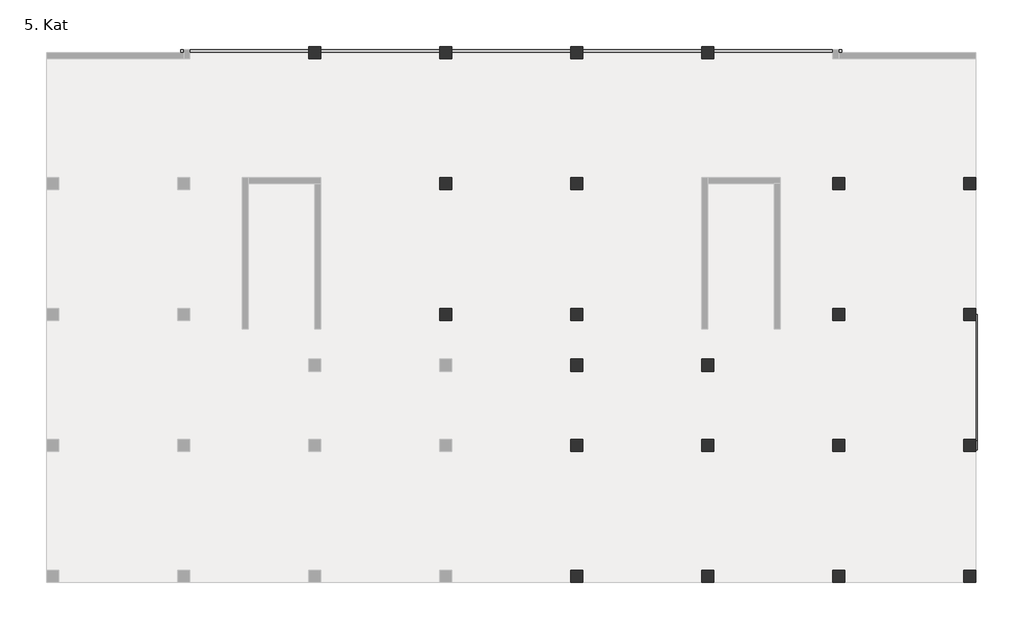
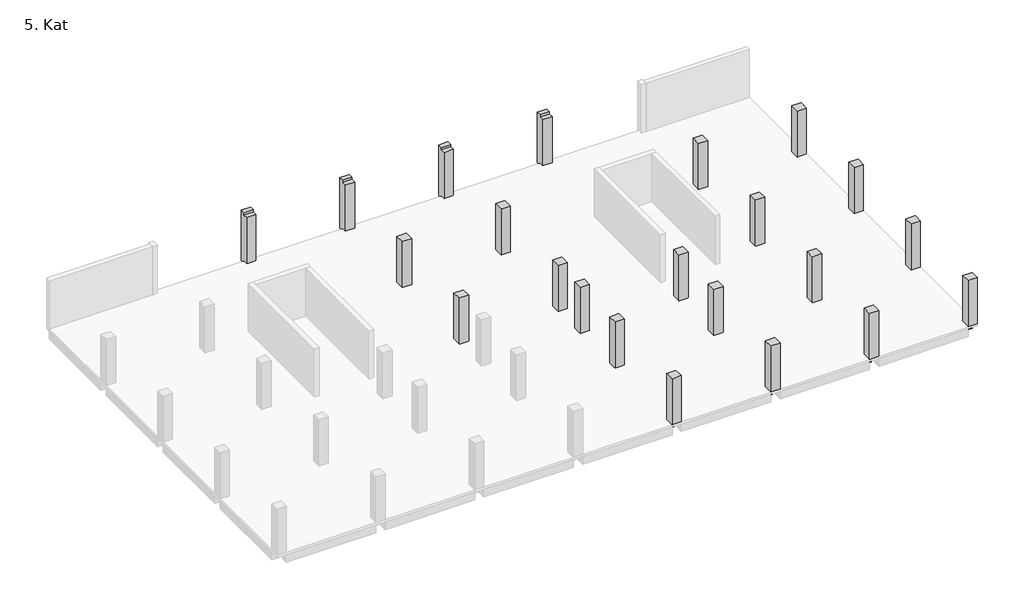
# One storey, part 2 of 2: 46 beams, 22 columns.
"""IFC4 building model written with IfcOpenShell, lengths in millimetres."""

from ifc_helpers import new_model, si_unit, frame, origin, place, context, project, spatial, polyline, outline, extrude, faceted_brep, element, save

model = new_model("IFC4")

# Units and contexts
model_context = context("Model", 3, world=origin())
ifc_project = project(units=[si_unit("LENGTHUNIT", "METRE", prefix="MILLI")], contexts=[model_context])

# Site, building, storey
site = spatial("IfcSite", under=ifc_project)
building = spatial("IfcBuilding", under=site)
storey = spatial("IfcBuildingStorey", under=building, Name="5. Kat", Elevation=26500.0)

# Beams
placement = place(None, origin())
element("IfcBeam", 1, ObjectType="M_Concrete-Rectangular Beam : 60x70cm kiriş", at=placement, inside=storey, context=model_context, shape_type="Brep", body=[
    faceted_brep([(8899.9995273, 34200.0000099, 26500.0), (8899.9993907, 33600.0000099, 26500.0), (16599.9993907, 33600.0000099, 26500.0), (16599.9993907, 34200.0000099, 26500.0), (8899.9993907, 33600.0000099, 25800.0), (16599.9993907, 33600.0000099, 25800.0), (8899.9995273, 34200.0000099, 25800.0), (16599.9993907, 34200.0000099, 25800.0)], [[[0, 1, 2, 3]], [[1, 4, 5, 2]], [[4, 6, 7, 5]], [[3, 7, 6, 0]], [[0, 6, 4, 1]], [[3, 2, 5, 7]]]),
])
element("IfcBeam", 2, ObjectType="M_Concrete-Rectangular Beam : 60x70cm kiriş", at=placement, inside=storey, context=model_context, shape_type="SweptSolid", body=[
    extrude(outline(polyline([(25099.9993907, 34200.0000277), (25099.9993907, 33600.0000277), (17399.9993907, 33600.0000277), (17399.9993907, 34200.0000277), (25099.9993907, 34200.0000277)])), frame((0.0, 0.0, 25800.0), z_axis=(0.0, 0.0, 1.0), x_axis=(1.0, 0.0, 0.0)), (0.0, 0.0, 1.0), 700.0),
])
element("IfcBeam", 3, ObjectType="M_Concrete-Rectangular Beam : 60x70cm kiriş", at=placement, inside=storey, context=model_context, shape_type="SweptSolid", body=[
    extrude(outline(polyline([(33599.9993907, 34200.000044), (33599.9993907, 33600.000044), (25899.9993907, 33600.000044), (25899.9993907, 34200.000044), (33599.9993907, 34200.000044)])), frame((0.0, 0.0, 25800.0), z_axis=(0.0, 0.0, 1.0), x_axis=(1.0, 0.0, 0.0)), (0.0, 0.0, 1.0), 700.0),
])
element("IfcBeam", 4, ObjectType="M_Concrete-Rectangular Beam : 60x70cm kiriş", at=placement, inside=storey, context=model_context, shape_type="SweptSolid", body=[
    extrude(outline(polyline([(34399.9993907, 33600.0000618), (34399.9993907, 34200.0000618), (42099.9993899, 34200.0000618), (42099.9993899, 33600.0000618), (34399.9993907, 33600.0000618)])), frame((0.0, 0.0, 25800.0), z_axis=(0.0, 0.0, 1.0), x_axis=(1.0, 0.0, 0.0)), (0.0, 0.0, 1.0), 700.0),
])
element("IfcBeam", 5, ObjectType="M_Concrete-Rectangular Beam : 60x70cm kiriş", at=placement, inside=storey, context=model_context, shape_type="Brep", body=[
    faceted_brep([(42899.999681, 34200.0000788, 26500.0), (42899.999681, 33600.0000788, 26500.0), (50599.9994944, 33600.0000788, 26500.0), (50599.9994944, 34000.0004303, 26500.0), (50599.9994944, 34193.7257565, 26500.0), (50999.9994944, 34193.7257565, 26500.0), (50999.9994944, 34200.0000788, 26500.0), (42899.999681, 34200.0000788, 25800.0), (50999.9994944, 34200.0000788, 25800.0), (42899.999681, 33600.0000788, 25800.0), (50999.9994944, 34193.7257565, 25800.0), (50599.9994944, 34193.7257565, 25800.0), (50599.9994944, 34000.0004303, 25800.0), (50599.9994944, 33600.0000788, 25800.0)], [[[0, 1, 2, 3, 4, 5, 6]], [[7, 0, 6, 8]], [[9, 7, 8, 10, 11, 12, 13]], [[1, 9, 13, 2]], [[1, 0, 7, 9]], [[8, 6, 5, 10]], [[11, 4, 3, 2, 13, 12]], [[4, 11, 10, 5]]]),
])
element("IfcBeam", 6, ObjectType="M_Concrete-Rectangular Beam : 60x70cm kiriş", at=placement, inside=storey, context=model_context, shape_type="Brep", body=[
    faceted_brep([(17399.9996817, 33600.0009197, 26500.0), (16799.9996817, 33600.0009197, 26500.0), (16799.9996817, 25900.0003816, 26500.0), (16999.9995362, 25900.0003816, 26500.0), (17399.9996817, 25900.0003816, 26500.0), (17399.9996817, 33600.0009197, 25800.0), (17399.9996817, 25900.0003816, 25800.0), (16799.9996817, 33600.0009197, 25800.0), (16799.9996817, 25900.0003816, 25800.0)], [[[0, 1, 2, 3, 4]], [[5, 0, 4, 6]], [[7, 5, 6, 8]], [[1, 7, 8, 2]], [[0, 5, 7, 1]], [[4, 3, 2, 8, 6]]]),
])
element("IfcBeam", 7, ObjectType="M_Concrete-Rectangular Beam : 60x70cm kiriş", at=placement, inside=storey, context=model_context, shape_type="SweptSolid", body=[
    extrude(outline(polyline([(25899.9996503, 25900.0004105), (25299.9996503, 25900.0004105), (25299.9996503, 33600.0009197), (25899.9996503, 33600.0009197), (25899.9996503, 25900.0004105)])), frame((0.0, 0.0, 25800.0), z_axis=(0.0, 0.0, 1.0), x_axis=(1.0, 0.0, 0.0)), (0.0, 0.0, 1.0), 700.0),
])
element("IfcBeam", 8, ObjectType="M_Concrete-Rectangular Beam : 60x70cm kiriş", at=placement, inside=storey, context=model_context, shape_type="Brep", body=[
    faceted_brep([(17399.9996817, 25900.0000279, 26500.0), (17399.9995847, 25500.0003816, 26500.0), (17399.9995362, 25300.0000279, 26500.0), (25099.9993907, 25300.0000279, 26500.0), (25099.9993907, 25900.0000279, 26500.0), (17399.9996817, 25900.0000279, 25800.0), (25099.9993907, 25900.0000279, 25800.0), (17399.9995362, 25300.0000279, 25800.0), (25099.9993907, 25300.0000279, 25800.0)], [[[0, 1, 2, 3, 4]], [[5, 0, 4, 6]], [[7, 5, 6, 8]], [[8, 3, 2, 7]], [[0, 5, 7, 2, 1]], [[3, 8, 6, 4]]]),
])
element("IfcBeam", 9, ObjectType="M_Concrete-Rectangular Beam : 40x70cm kiriş 2", at=placement, inside=storey, context=model_context, shape_type="SweptSolid", body=[
    extrude(outline(polyline([(25099.999715, 17400.0003766), (25099.999715, 17000.0003766), (17399.9995362, 17000.0003766), (17399.9995362, 17400.0003766), (25099.999715, 17400.0003766)])), frame((0.0, 0.0, 25800.0), z_axis=(0.0, 0.0, 1.0), x_axis=(1.0, 0.0, 0.0)), (0.0, 0.0, 1.0), 700.0),
])
element("IfcBeam", 10, ObjectType="M_Concrete-Rectangular Beam : 60x70cm kiriş", at=placement, inside=storey, context=model_context, shape_type="SweptSolid", body=[
    extrude(outline(polyline([(25299.999682, 25099.9999518), (25899.999682, 25099.9999518), (25899.999682, 17400.0009197), (25299.999682, 17400.0009197), (25299.999682, 25099.9999518)])), frame((0.0, 0.0, 25800.0), z_axis=(0.0, 0.0, 1.0), x_axis=(1.0, 0.0, 0.0)), (0.0, 0.0, 1.0), 700.0),
])
element("IfcBeam", 11, ObjectType="M_Concrete-Rectangular Beam : 60x70cm kiriş", at=placement, inside=storey, context=model_context, shape_type="Brep", body=[
    faceted_brep([(25899.9996503, 25900.0003995, 26500.0), (25899.9993907, 25300.0003995, 26500.0), (33599.9993907, 25300.0003995, 26500.0), (33599.9993907, 25900.0003995, 26500.0), (25899.9996503, 25900.0003995, 25800.0), (33599.9993907, 25900.0003995, 25800.0), (25899.9993907, 25300.0003995, 25800.0), (33599.9993907, 25300.0003995, 25800.0)], [[[0, 1, 2, 3]], [[4, 0, 3, 5]], [[6, 4, 5, 7]], [[1, 6, 7, 2]], [[0, 4, 6, 1]], [[3, 2, 7, 5]]]),
])
element("IfcBeam", 12, ObjectType="M_Concrete-Rectangular Beam : 60x70cm kiriş", at=placement, inside=storey, context=model_context, shape_type="Brep", body=[
    faceted_brep([(34199.9994248, 33600.0009197, 26500.0), (33599.9994248, 33600.000044, 26500.0), (33599.9994248, 25900.0003995, 26500.0), (34199.9994248, 25900.0004105, 26500.0), (33599.9994248, 33600.000044, 25800.0), (33599.9994248, 25900.0003995, 25800.0), (34199.9994248, 33600.0009197, 25800.0), (34199.9994248, 25900.0004105, 25800.0)], [[[0, 1, 2, 3]], [[1, 4, 5, 2]], [[4, 6, 7, 5]], [[3, 7, 6, 0]], [[0, 6, 4, 1]], [[2, 5, 7, 3]]]),
])
element("IfcBeam", 13, ObjectType="M_Concrete-Rectangular Beam : 60x70cm kiriş", at=placement, inside=storey, context=model_context, shape_type="Brep", body=[
    faceted_brep([(34399.9993907, 25900.0004179, 26500.0), (34399.9993907, 25300.0004179, 26500.0), (42099.9995162, 25300.0004179, 26500.0), (42099.9995162, 25500.0004459, 26500.0), (42099.9995162, 25900.0004179, 26500.0), (34399.9993907, 25300.0004179, 25800.0), (42099.9995162, 25300.0004179, 25800.0), (34399.9993907, 25900.0004179, 25800.0), (42099.9995162, 25900.0004179, 25800.0)], [[[0, 1, 2, 3, 4]], [[1, 5, 6, 2]], [[5, 7, 8, 6]], [[7, 0, 4, 8]], [[5, 1, 0, 7]], [[4, 3, 2, 6, 8]]]),
])
element("IfcBeam", 14, ObjectType="M_Concrete-Rectangular Beam : 60x70cm kiriş", at=placement, inside=storey, context=model_context, shape_type="Brep", body=[
    faceted_brep([(42099.9994393, 25900.0004179, 26500.0), (42499.9995162, 25900.0004366, 26500.0), (42699.9994393, 25900.0004459, 26500.0), (42699.9994393, 33600.0009197, 26500.0), (42099.9994393, 33600.0000618, 26500.0), (42099.9994393, 25900.0004179, 25800.0), (42099.9994393, 33600.0000618, 25800.0), (42699.9994393, 25900.0004459, 25800.0), (42699.9994393, 33600.0009197, 25800.0)], [[[0, 1, 2, 3, 4]], [[5, 0, 4, 6]], [[7, 5, 6, 8]], [[8, 3, 2, 7]], [[0, 5, 7, 2, 1]], [[6, 4, 3, 8]]]),
])
element("IfcBeam", 15, ObjectType="M_Concrete-Rectangular Beam : 60x70cm kiriş", at=placement, inside=storey, context=model_context, shape_type="Brep", body=[
    faceted_brep([(50599.9993899, 25300.0004722, 26500.0), (50599.9993899, 25900.0004722, 26500.0), (47199.999381, 25900.0004722, 26500.0), (47199.999381, 25500.0004459, 26500.0), (47199.999381, 25300.0004722, 26500.0), (50599.9993899, 25900.0004722, 25800.0), (47199.999381, 25900.0004722, 25800.0), (50599.9993899, 25300.0004722, 25800.0), (47199.999381, 25300.0004722, 25800.0)], [[[0, 1, 2, 3, 4]], [[1, 5, 6, 2]], [[5, 7, 8, 6]], [[7, 0, 4, 8]], [[5, 1, 0, 7]], [[8, 4, 3, 2, 6]]]),
])
element("IfcBeam", 16, ObjectType="M_Concrete-Rectangular Beam : 60x70cm kiriş", at=placement, inside=storey, context=model_context, shape_type="Brep", body=[
    faceted_brep([(51199.9994348, 33600.0004303, 26500.0), (50999.9994944, 33600.0003131, 26500.0), (50599.9994348, 33600.0000788, 26500.0), (50599.9994348, 25900.0004722, 26500.0), (51199.9994348, 25899.9999188, 26500.0), (51199.9994348, 25899.9999188, 25800.0), (51199.9994348, 33600.0004303, 25800.0), (50599.9994348, 33600.0000788, 25800.0), (50599.9994348, 25900.0004722, 25800.0)], [[[0, 1, 2, 3, 4]], [[4, 5, 6, 0]], [[7, 6, 5, 8]], [[2, 7, 8, 3]], [[0, 6, 7, 2, 1]], [[3, 8, 5, 4]]]),
])
element("IfcBeam", 17, ObjectType="M_Concrete-Rectangular Beam : 60x70cm kiriş", at=placement, inside=storey, context=model_context, shape_type="SweptSolid", body=[
    extrude(outline(polyline([(59100.0000836, 25900.0000972), (59100.0000836, 25300.0000972), (51399.9996879, 25300.0000972), (51399.9996879, 25900.0000972), (59100.0000836, 25900.0000972)])), frame((0.0, 0.0, 25800.0), z_axis=(0.0, 0.0, 1.0), x_axis=(1.0, 0.0, 0.0)), (0.0, 0.0, 1.0), 700.0),
])
element("IfcBeam", 18, ObjectType="M_Concrete-Rectangular Beam : 60x70cm kiriş", at=placement, inside=storey, context=model_context, shape_type="SweptSolid", body=[
    extrude(outline(polyline([(59899.9996867, 25900.0004522), (59299.9996867, 25900.0004522), (59299.9996867, 33600.0004303), (59899.9996867, 33600.0004303), (59899.9996867, 25900.0004522)])), frame((0.0, 0.0, 25800.0), z_axis=(0.0, 0.0, 1.0), x_axis=(1.0, 0.0, 0.0)), (0.0, 0.0, 1.0), 700.0),
])
element("IfcBeam", 19, ObjectType="M_Concrete-Rectangular Beam : 60x70cm kiriş", at=placement, inside=storey, context=model_context, shape_type="SweptSolid", body=[
    extrude(outline(polyline([(33599.9994953, 25100.0004105), (34199.9994953, 25100.0004105), (34199.9994953, 17400.0009197), (33599.9994953, 17400.0009197), (33599.9994953, 25100.0004105)])), frame((0.0, 0.0, 25800.0), z_axis=(0.0, 0.0, 1.0), x_axis=(1.0, 0.0, 0.0)), (0.0, 0.0, 1.0), 700.0),
])
element("IfcBeam", 20, ObjectType="M_Concrete-Rectangular Beam : 40x70cm kiriş 2", at=placement, inside=storey, context=model_context, shape_type="Brep", body=[
    faceted_brep([(25899.999682, 17400.0007711, 26500.0), (25899.9993907, 17000.0007711, 26500.0), (33599.9993907, 17000.0007711, 26500.0), (33599.9994953, 17400.0007711, 26500.0), (33599.9993907, 17000.0007711, 25800.0), (25899.9993907, 17000.0007711, 25800.0), (25899.999682, 17400.0007711, 25800.0), (33599.9994953, 17400.0007711, 25800.0)], [[[0, 1, 2, 3]], [[4, 2, 1, 5]], [[5, 6, 7, 4]], [[6, 0, 3, 7]], [[0, 6, 5, 1]], [[7, 3, 2, 4]]]),
])
element("IfcBeam", 21, ObjectType="M_Concrete-Rectangular Beam : 40x70cm kiriş 2", at=placement, inside=storey, context=model_context, shape_type="SweptSolid", body=[
    extrude(outline(polyline([(42499.9995162, 14100.0003816), (42099.9995162, 14100.0003816), (42099.9995162, 16050.0004138), (42499.9995162, 16050.0004138), (42499.9995162, 14100.0003816)])), frame((0.0, 0.0, 25800.0), z_axis=(0.0, 0.0, 1.0), x_axis=(1.0, 0.0, 0.0)), (0.0, 0.0, 1.0), 700.0),
])
element("IfcBeam", 22, ObjectType="M_Concrete-Rectangular Beam : 40x70cm kiriş 2", at=placement, inside=storey, context=model_context, shape_type="SweptSolid", body=[
    extrude(outline(polyline([(34399.9997415, 13300.0003995), (34399.9997415, 13700.0003995), (41999.9997966, 13700.0003995), (41999.9997966, 13300.0003995), (34399.9997415, 13300.0003995)])), frame((0.0, 0.0, 25800.0), z_axis=(0.0, 0.0, 1.0), x_axis=(1.0, 0.0, 0.0)), (0.0, 0.0, 1.0), 700.0),
])
element("IfcBeam", 23, ObjectType="M_Concrete-Rectangular Beam : 40x70cm kiriş 2", at=placement, inside=storey, context=model_context, shape_type="SweptSolid", body=[
    extrude(outline(polyline([(34399.9993907, 17000.0007895), (34399.9993907, 17400.0007895), (42099.9995162, 17400.0007895), (42099.9995162, 17000.0007895), (34399.9993907, 17000.0007895)])), frame((0.0, 0.0, 25800.0), z_axis=(0.0, 0.0, 1.0), x_axis=(1.0, 0.0, 0.0)), (0.0, 0.0, 1.0), 700.0),
])
element("IfcBeam", 24, ObjectType="M_Concrete-Rectangular Beam : 40x70cm kiriş 2", at=placement, inside=storey, context=model_context, shape_type="SweptSolid", body=[
    extrude(outline(polyline([(42499.9995162, 17000.0003766), (42499.9995162, 17400.0003766), (46799.999381, 17400.0003766), (46799.999381, 17000.0003766), (42499.9995162, 17000.0003766)])), frame((0.0, 0.0, 25800.0), z_axis=(0.0, 0.0, 1.0), x_axis=(1.0, 0.0, 0.0)), (0.0, 0.0, 1.0), 700.0),
])
element("IfcBeam", 25, ObjectType="M_Concrete-Rectangular Beam : 60x70cm kiriş", at=placement, inside=storey, context=model_context, shape_type="SweptSolid", body=[
    extrude(outline(polyline([(34199.9997451, 14100.0003995), (33599.9997451, 14100.0003995), (33599.9997451, 16599.9999518), (34199.9997451, 16599.9999518), (34199.9997451, 14100.0003995)])), frame((0.0, 0.0, 25800.0), z_axis=(0.0, 0.0, 1.0), x_axis=(1.0, 0.0, 0.0)), (0.0, 0.0, 1.0), 700.0),
])
element("IfcBeam", 26, ObjectType="M_Concrete-Rectangular Beam : 40x70cm kiriş 2", at=placement, inside=storey, context=model_context, shape_type="Brep", body=[
    faceted_brep([(42899.9990901, 13700.0003995, 26500.0), (42899.9990901, 13300.0003995, 26500.0), (46799.999381, 13300.0003995, 26500.0), (47199.999381, 13300.0003995, 26500.0), (50599.9996909, 13300.0003995, 26500.0), (50599.9996909, 13700.0003995, 26500.0), (47199.999381, 13700.0003995, 26500.0), (46799.999381, 13700.0003995, 26500.0), (42899.9990901, 13300.0003995, 25800.0), (46799.999381, 13300.0003995, 25800.0), (47199.999381, 13300.0003995, 25800.0), (50599.9996909, 13300.0003995, 25800.0), (42899.9990901, 13700.0003995, 25800.0), (46799.999381, 13700.0003995, 25800.0), (47199.999381, 13700.0003995, 25800.0), (50599.9996909, 13700.0003995, 25800.0)], [[[0, 1, 2, 3, 4, 5, 6, 7]], [[1, 8, 9, 10, 11, 4, 3, 2]], [[8, 12, 13, 14, 15, 11, 10, 9]], [[12, 0, 7, 6, 5, 15, 14, 13]], [[5, 4, 11, 15]], [[0, 12, 8, 1]]]),
])
element("IfcBeam", 27, ObjectType="M_Concrete-Rectangular Beam : 40x70cm kiriş 2", at=placement, inside=storey, context=model_context, shape_type="SweptSolid", body=[
    extrude(outline(polyline([(46799.999381, 16050.0004138), (47199.999381, 16050.0004138), (47199.999381, 13700.0003995), (46799.999381, 13700.0003995), (46799.999381, 16050.0004138)])), frame((0.0, 0.0, 25800.0), z_axis=(0.0, 0.0, 1.0), x_axis=(1.0, 0.0, 0.0)), (0.0, 0.0, 1.0), 700.0),
    extrude(outline(polyline([(46799.999381, 13300.0003995), (47199.999381, 13300.0003995), (47199.999381, 8800.0009197), (46799.999381, 8800.0009197), (46799.999381, 13300.0003995)])), frame((0.0, 0.0, 25800.0), z_axis=(0.0, 0.0, 1.0), x_axis=(1.0, 0.0, 0.0)), (0.0, 0.0, 1.0), 700.0),
])
element("IfcBeam", 28, ObjectType="M_Concrete-Rectangular Beam : 60x70cm kiriş", at=placement, inside=storey, context=model_context, shape_type="Brep", body=[
    faceted_brep([(34399.9993907, 8800.0009197, 26500.0), (34399.9993907, 8200.0009197, 26500.0), (42099.9993899, 8200.0009197, 26500.0), (42099.9993899, 8800.0009197, 26500.0), (41999.9997966, 8800.0009197, 26500.0), (34399.9993907, 8200.0009197, 25800.0), (42099.9993899, 8200.0009197, 25800.0), (34399.9993907, 8800.0009197, 25800.0), (41999.9997966, 8800.0009197, 25800.0), (42099.9993899, 8800.0009197, 25800.0)], [[[0, 1, 2, 3, 4]], [[1, 5, 6, 2]], [[5, 7, 8, 9, 6]], [[7, 0, 4, 3, 9, 8]], [[5, 1, 0, 7]], [[3, 2, 6, 9]]]),
])
element("IfcBeam", 29, ObjectType="M_Concrete-Rectangular Beam : 60x70cm kiriş", at=placement, inside=storey, context=model_context, shape_type="Brep", body=[
    faceted_brep([(50599.9993899, 8200.0009197, 26500.0), (50599.9993899, 8800.0009197, 26500.0), (47199.999381, 8800.0009197, 26500.0), (46799.999381, 8800.0009197, 26500.0), (42899.9993899, 8800.0009197, 26500.0), (42899.9993899, 8200.0009197, 26500.0), (50599.9993899, 8200.0009197, 25800.0), (42899.9993899, 8200.0009197, 25800.0), (50599.9993899, 8800.0009197, 25800.0), (42899.9993899, 8800.0009197, 25800.0), (46799.999381, 8800.0009197, 25800.0), (47199.999381, 8800.0009197, 25800.0)], [[[0, 1, 2, 3, 4, 5]], [[6, 0, 5, 7]], [[8, 6, 7, 9, 10, 11]], [[1, 8, 11, 10, 9, 4, 3, 2]], [[0, 6, 8, 1]], [[5, 4, 9, 7]]]),
])
element("IfcBeam", 30, ObjectType="M_Concrete-Rectangular Beam : 60x70cm kiriş", at=placement, inside=storey, context=model_context, shape_type="Brep", body=[
    faceted_brep([(41999.9997966, 13700.0003995, 26500.0), (41999.9997966, 13300.0003995, 26500.0), (41999.9997966, 8800.0009197, 26500.0), (42099.9993899, 8800.0009197, 26500.0), (42099.9993899, 8900.0009197, 26500.0), (42599.9997966, 8900.0009197, 26500.0), (42599.9997966, 13300.0003816, 26500.0), (42099.9993899, 13300.0003816, 26500.0), (42099.9993899, 13700.0003995, 26500.0), (42599.9997966, 8900.0009197, 25800.0), (42599.9997966, 13300.0003816, 25800.0), (41999.9997966, 8800.0009197, 25800.0), (41999.9997966, 13300.0003995, 25800.0), (41999.9997966, 13700.0003995, 25800.0), (42099.9993899, 13700.0003995, 25800.0), (42099.9993899, 13300.0003816, 25800.0), (42099.9993899, 8900.0009197, 25800.0), (42099.9993899, 8800.0009197, 25800.0)], [[[0, 1, 2, 3, 4, 5, 6, 7, 8]], [[5, 9, 10, 6]], [[11, 12, 13, 14, 15, 10, 9, 16, 17]], [[11, 2, 1, 0, 13, 12]], [[2, 11, 17, 3]], [[13, 0, 8, 14]], [[16, 4, 3, 17]], [[4, 16, 9, 5]], [[15, 7, 6, 10]], [[7, 15, 14, 8]]]),
])
element("IfcBeam", 31, ObjectType="M_Concrete-Rectangular Beam : 60x70cm kiriş", at=placement, inside=storey, context=model_context, shape_type="SweptSolid", body=[
    extrude(outline(polyline([(34199.9994953, 8900.0009197), (33599.9994953, 8900.0009197), (33599.9994953, 13300.0003995), (34199.9994953, 13300.0003995), (34199.9994953, 8900.0009197)])), frame((0.0, 0.0, 25800.0), z_axis=(0.0, 0.0, 1.0), x_axis=(1.0, 0.0, 0.0)), (0.0, 0.0, 1.0), 700.0),
])
element("IfcBeam", 32, ObjectType="M_Concrete-Rectangular Beam : 60x70cm kiriş", at=placement, inside=storey, context=model_context, shape_type="SweptSolid", body=[
    extrude(outline(polyline([(47199.999381, 16800.0008288), (47199.999381, 17400.0008288), (50599.9993899, 17400.0008288), (50599.9993899, 16800.0008288), (47199.999381, 16800.0008288)])), frame((0.0, 0.0, 25800.0), z_axis=(0.0, 0.0, 1.0), x_axis=(1.0, 0.0, 0.0)), (0.0, 0.0, 1.0), 700.0),
])
element("IfcBeam", 33, ObjectType="M_Concrete-Rectangular Beam : 60x70cm kiriş", at=placement, inside=storey, context=model_context, shape_type="Brep", body=[
    faceted_brep([(50599.999688, 17400.0008288, 26500.0), (51199.999688, 17400.0009197, 26500.0), (51199.999688, 25099.9999414, 26500.0), (50599.999688, 25099.9999414, 26500.0), (50599.999688, 17400.0008288, 25800.0), (50599.999688, 25099.9999414, 25800.0), (51199.999688, 17400.0009197, 25800.0), (51199.999688, 25099.9999414, 25800.0)], [[[0, 1, 2, 3]], [[4, 0, 3, 5]], [[6, 4, 5, 7]], [[7, 2, 1, 6]], [[0, 4, 6, 1]], [[2, 7, 5, 3]]]),
])
element("IfcBeam", 34, ObjectType="M_Concrete-Rectangular Beam : 60x70cm kiriş", at=placement, inside=storey, context=model_context, shape_type="SweptSolid", body=[
    extrude(outline(polyline([(59899.9997153, 17400.0009197), (59299.9997153, 17400.0009197), (59299.9997153, 25099.9999188), (59899.9997153, 25099.9999188), (59899.9997153, 17400.0009197)])), frame((0.0, 0.0, 25800.0), z_axis=(0.0, 0.0, 1.0), x_axis=(1.0, 0.0, 0.0)), (0.0, 0.0, 1.0), 700.0),
])
element("IfcBeam", 35, ObjectType="M_Concrete-Rectangular Beam : 60x70cm kiriş", at=placement, inside=storey, context=model_context, shape_type="SweptSolid", body=[
    extrude(outline(polyline([(51399.9993899, 16799.9995872), (51399.9993899, 17399.9995872), (59100.0000836, 17399.9995872), (59100.0000836, 16799.9995872), (51399.9993899, 16799.9995872)])), frame((0.0, 0.0, 25800.0), z_axis=(0.0, 0.0, 1.0), x_axis=(1.0, 0.0, 0.0)), (0.0, 0.0, 1.0), 700.0),
])
element("IfcBeam", 36, ObjectType="M_Concrete-Rectangular Beam : 60x70cm kiriş", at=placement, inside=storey, context=model_context, shape_type="Brep", body=[
    faceted_brep([(50599.9996909, 8900.000455, 26500.0), (51199.9996909, 8900.000455, 26500.0), (51199.9996909, 16600.0009197, 26500.0), (50599.9996909, 16600.0009197, 26500.0), (50599.9996909, 13700.0003995, 26500.0), (50599.9996909, 13300.0003995, 26500.0), (50599.9996909, 8900.000455, 25800.0), (50599.9996909, 16600.0009197, 25800.0), (50599.9996909, 13700.0003995, 25800.0), (50599.9996909, 13300.0003995, 25800.0), (51199.9996909, 8900.000455, 25800.0), (51199.9996909, 16600.0009197, 25800.0)], [[[0, 1, 2, 3, 4, 5]], [[6, 0, 5, 4, 3, 7, 8, 9]], [[10, 6, 9, 8, 7, 11]], [[1, 10, 11, 2]], [[1, 0, 6, 10]], [[2, 11, 7, 3]]]),
])
element("IfcBeam", 37, ObjectType="M_Concrete-Rectangular Beam : 60x70cm kiriş", at=placement, inside=storey, context=model_context, shape_type="SweptSolid", body=[
    extrude(outline(polyline([(59999.9993848, 8800.0009197), (59999.9993848, 8200.0009197), (59900.0000836, 8200.0009197), (59900.0000836, 8800.0009197), (59999.9993848, 8800.0009197)])), frame((0.0, 0.0, 25800.0), z_axis=(0.0, 0.0, 1.0), x_axis=(1.0, 0.0, 0.0)), (0.0, 0.0, 1.0), 700.0),
    extrude(outline(polyline([(51399.9993899, 8200.0009197), (51399.9993899, 8800.0009197), (59100.0000836, 8800.0009197), (59100.0000836, 8200.0009197), (51399.9993899, 8200.0009197)])), frame((0.0, 0.0, 25800.0), z_axis=(0.0, 0.0, 1.0), x_axis=(1.0, 0.0, 0.0)), (0.0, 0.0, 1.0), 700.0),
])
element("IfcBeam", 38, ObjectType="M_Concrete-Rectangular Beam : 60x70cm kiriş", at=placement, inside=storey, context=model_context, shape_type="SweptSolid", body=[
    extrude(outline(polyline([(59999.9993848, 17000.0009197), (59999.9993848, 8800.0009197), (59900.0000836, 8800.0009197), (59900.0000836, 8900.0009197), (59399.9993848, 8900.0009197), (59399.9993848, 16600.0009197), (59900.0000836, 16600.0009197), (59900.0000836, 17000.0009197), (59999.9993848, 17000.0009197)])), frame((0.0, 0.0, 25800.0), z_axis=(0.0, 0.0, 1.0), x_axis=(1.0, 0.0, 0.0)), (0.0, 0.0, 1.0), 700.0),
])
element("IfcBeam", 39, ObjectType="M_Concrete-Rectangular Beam : 60x70cm kiriş", at=placement, inside=storey, context=model_context, shape_type="SweptSolid", body=[
    extrude(outline(polyline([(59899.9997503, 400.0009197), (59299.9997503, 400.0009197), (59299.9997503, 8100.0009197), (59899.9997503, 8100.0009197), (59899.9997503, 400.0009197)])), frame((0.0, 0.0, 25800.0), z_axis=(0.0, 0.0, 1.0), x_axis=(1.0, 0.0, 0.0)), (0.0, 0.0, 1.0), 700.0),
])
element("IfcBeam", 40, ObjectType="M_Concrete-Rectangular Beam : 60x70cm kiriş", at=placement, inside=storey, context=model_context, shape_type="SweptSolid", body=[
    extrude(outline(polyline([(51199.999723, 400.0009197), (50599.999723, 400.0009197), (50599.999723, 8100.0009197), (51199.999723, 8100.0009197), (51199.999723, 400.0009197)])), frame((0.0, 0.0, 25800.0), z_axis=(0.0, 0.0, 1.0), x_axis=(1.0, 0.0, 0.0)), (0.0, 0.0, 1.0), 700.0),
])
element("IfcBeam", 41, ObjectType="M_Concrete-Rectangular Beam : 60x70cm kiriş", at=placement, inside=storey, context=model_context, shape_type="SweptSolid", body=[
    extrude(outline(polyline([(42699.999723, 400.0009197), (42099.999723, 400.0009197), (42099.999723, 8100.0009197), (42699.999723, 8100.0009197), (42699.999723, 400.0009197)])), frame((0.0, 0.0, 25800.0), z_axis=(0.0, 0.0, 1.0), x_axis=(1.0, 0.0, 0.0)), (0.0, 0.0, 1.0), 700.0),
])
element("IfcBeam", 42, ObjectType="M_Concrete-Rectangular Beam : 60x70cm kiriş", at=placement, inside=storey, context=model_context, shape_type="SweptSolid", body=[
    extrude(outline(polyline([(34199.9997451, 400.0004179), (33599.9997451, 400.0004179), (33599.9997451, 8100.0004174), (34199.9997451, 8100.0004174), (34199.9997451, 400.0004179)])), frame((0.0, 0.0, 25800.0), z_axis=(0.0, 0.0, 1.0), x_axis=(1.0, 0.0, 0.0)), (0.0, 0.0, 1.0), 700.0),
])
element("IfcBeam", 43, ObjectType="M_Concrete-Rectangular Beam : 60x70cm kiriş", at=placement, inside=storey, context=model_context, shape_type="SweptSolid", body=[
    extrude(outline(polyline([(8499.9995273, 34000.0004302), (8299.9993907, 34000.0004302), (8299.9993907, 34200.0000099), (8499.9995273, 34200.0000099), (8499.9995273, 34000.0004302)])), frame((0.0, 0.0, 25800.0), z_axis=(0.0, 0.0, 1.0), x_axis=(1.0, 0.0, 0.0)), (0.0, 0.0, 1.0), 700.0),
])
element("IfcBeam", 44, ObjectType="M_Concrete-Rectangular Beam : 60x70cm kiriş", at=placement, inside=storey, context=model_context, shape_type="SweptSolid", body=[
    extrude(outline(polyline([(16799.9996817, 25300.0000279), (16799.9996817, 25500.0003816), (16999.9995362, 25500.0003816), (16999.9995362, 25300.0000279), (16799.9996817, 25300.0000279)])), frame((0.0, 0.0, 25800.0), z_axis=(0.0, 0.0, 1.0), x_axis=(1.0, 0.0, 0.0)), (0.0, 0.0, 1.0), 700.0),
])
element("IfcBeam", 45, ObjectType="M_Concrete-Rectangular Beam : 60x70cm kiriş", at=placement, inside=storey, context=model_context, shape_type="SweptSolid", body=[
    extrude(outline(polyline([(42699.9994393, 25300.0004179), (42499.9995162, 25300.0004179), (42499.9995162, 25500.0004459), (42699.9994393, 25500.0004459), (42699.9994393, 25300.0004179)])), frame((0.0, 0.0, 25800.0), z_axis=(0.0, 0.0, 1.0), x_axis=(1.0, 0.0, 0.0)), (0.0, 0.0, 1.0), 700.0),
])
element("IfcBeam", 46, ObjectType="M_Concrete-Rectangular Beam : 60x70cm kiriş", at=placement, inside=storey, context=model_context, shape_type="Brep", body=[
    faceted_brep([(51199.9994348, 34200.0000788, 26500.0), (50999.9994944, 34200.0000788, 26500.0), (50999.9994944, 34193.7257565, 26500.0), (50999.9994944, 34000.0004303, 26500.0), (51199.9994348, 34000.0004303, 26500.0), (51199.9994348, 34200.0000788, 25800.0), (51199.9994348, 34000.0004303, 25800.0), (50999.9994944, 34000.0004303, 25800.0), (50999.9994944, 34193.7257565, 25800.0), (50999.9994944, 34200.0000788, 25800.0)], [[[0, 1, 2, 3, 4]], [[5, 0, 4, 6]], [[6, 7, 8, 9, 5]], [[0, 5, 9, 1]], [[7, 3, 2, 1, 9, 8]], [[6, 4, 3, 7]]]),
])

# Columns
element("IfcColumn", 47, ObjectType="M_Concrete-Rectangular-Column : 80x80cm kolon", at=placement, inside=storey, context=model_context, shape_type="SweptSolid", body=[
    extrude(outline(polyline([(34399.9993907, 400.0009197), (34399.9993907, -399.9990803), (33599.9993907, -399.9990803), (33599.9993907, 400.0009197), (34399.9993907, 400.0009197)])), frame((0.0, 0.0, 26700.0), z_axis=(0.0, 0.0, 1.0), x_axis=(1.0, 0.0, 0.0)), (0.0, 0.0, 1.0), 4200.0),
])
element("IfcColumn", 48, ObjectType="M_Concrete-Rectangular-Column : 80x80cm kolon", at=placement, inside=storey, context=model_context, shape_type="SweptSolid", body=[
    extrude(outline(polyline([(34399.9993907, 8900.0009197), (34399.9993907, 8100.0009197), (33599.9993907, 8100.0009197), (33599.9993907, 8900.0009197), (34399.9993907, 8900.0009197)])), frame((0.0, 0.0, 26700.0), z_axis=(0.0, 0.0, 1.0), x_axis=(1.0, 0.0, 0.0)), (0.0, 0.0, 1.0), 4200.0),
])
element("IfcColumn", 49, ObjectType="M_Concrete-Rectangular-Column : 80x80cm kolon", at=placement, inside=storey, context=model_context, shape_type="SweptSolid", body=[
    extrude(outline(polyline([(34399.9993907, 14100.0003995), (34399.9993907, 13300.0003995), (33599.9993907, 13300.0003995), (33599.9993907, 14100.0003995), (34399.9993907, 14100.0003995)])), frame((0.0, 0.0, 26700.0), z_axis=(0.0, 0.0, 1.0), x_axis=(1.0, 0.0, 0.0)), (0.0, 0.0, 1.0), 4200.0),
])
element("IfcColumn", 50, ObjectType="M_Concrete-Rectangular-Column : 80x80cm kolon", at=placement, inside=storey, context=model_context, shape_type="SweptSolid", body=[
    extrude(outline(polyline([(34399.9993907, 17400.0009197), (34399.9993907, 16600.0009197), (33599.9993907, 16600.0009197), (33599.9993907, 17400.0009197), (34399.9993907, 17400.0009197)])), frame((0.0, 0.0, 26700.0), z_axis=(0.0, 0.0, 1.0), x_axis=(1.0, 0.0, 0.0)), (0.0, 0.0, 1.0), 4200.0),
])
element("IfcColumn", 51, ObjectType="M_Concrete-Rectangular-Column : 80x80cm kolon", at=placement, inside=storey, context=model_context, shape_type="SweptSolid", body=[
    extrude(outline(polyline([(25899.9993907, 17400.0009197), (25899.9993907, 16600.0009197), (25099.9993907, 16600.0009197), (25099.9993907, 17400.0009197), (25899.9993907, 17400.0009197)])), frame((0.0, 0.0, 26700.0), z_axis=(0.0, 0.0, 1.0), x_axis=(1.0, 0.0, 0.0)), (0.0, 0.0, 1.0), 4200.0),
])
element("IfcColumn", 52, ObjectType="M_Concrete-Rectangular-Column : 80x80cm kolon", at=placement, inside=storey, context=model_context, shape_type="SweptSolid", body=[
    extrude(outline(polyline([(25899.9993907, 25900.0004105), (25899.9993907, 25100.0004105), (25099.9993907, 25100.0004105), (25099.9993907, 25900.0004105), (25899.9993907, 25900.0004105)])), frame((0.0, 0.0, 26700.0), z_axis=(0.0, 0.0, 1.0), x_axis=(1.0, 0.0, 0.0)), (0.0, 0.0, 1.0), 4200.0),
])
element("IfcColumn", 53, ObjectType="M_Concrete-Rectangular-Column : 80x80cm kolon", at=placement, inside=storey, context=model_context, shape_type="SweptSolid", body=[
    extrude(outline(polyline([(34399.9993907, 25900.0004105), (34399.9993907, 25100.0004105), (33599.9993907, 25100.0004105), (33599.9993907, 25900.0004105), (34399.9993907, 25900.0004105)])), frame((0.0, 0.0, 26700.0), z_axis=(0.0, 0.0, 1.0), x_axis=(1.0, 0.0, 0.0)), (0.0, 0.0, 1.0), 4200.0),
])
element("IfcColumn", 54, ObjectType="M_Concrete-Rectangular-Column : 80x80cm kolon", at=placement, inside=storey, context=model_context, shape_type="SweptSolid", body=[
    extrude(outline(polyline([(34400.0009197, 31100.0), (34400.0009197, 26500.0), (34000.0004302, 26500.0), (34000.0004302, 26700.0), (33600.0009197, 26700.0), (33600.0009197, 30900.0), (34000.0004302, 30900.0), (34000.0004302, 31100.0), (34400.0009197, 31100.0)])), frame((33599.9993907, 0.0, 0.0), z_axis=(1.0, 0.0, 0.0), x_axis=(0.0, 1.0, 0.0)), (0.0, 0.0, 1.0), 800.0),
])
element("IfcColumn", 55, ObjectType="M_Concrete-Rectangular-Column : 80x80cm kolon", at=placement, inside=storey, context=model_context, shape_type="SweptSolid", body=[
    extrude(outline(polyline([(34400.0009197, 31100.0), (34400.0009197, 26500.0), (34000.0004302, 26500.0), (34000.0004302, 26700.0), (33600.0009197, 26700.0), (33600.0009197, 30900.0), (34000.0004302, 30900.0), (34000.0004302, 31100.0), (34400.0009197, 31100.0)])), frame((25099.9993907, 0.0, 0.0), z_axis=(1.0, 0.0, 0.0), x_axis=(0.0, 1.0, 0.0)), (0.0, 0.0, 1.0), 800.0),
])
element("IfcColumn", 56, ObjectType="M_Concrete-Rectangular-Column : 80x80cm kolon", at=placement, inside=storey, context=model_context, shape_type="SweptSolid", body=[
    extrude(outline(polyline([(34400.0009197, 31100.0), (34400.0009197, 26500.0), (34000.0004302, 26500.0), (34000.0004302, 26700.0), (33600.0009197, 26700.0), (33600.0009197, 30900.0), (34000.0004302, 30900.0), (34000.0004302, 31100.0), (34400.0009197, 31100.0)])), frame((16599.9993907, 0.0, 0.0), z_axis=(1.0, 0.0, 0.0), x_axis=(0.0, 1.0, 0.0)), (0.0, 0.0, 1.0), 800.0),
])
element("IfcColumn", 57, ObjectType="M_Concrete-Rectangular-Column : 80x80cm kolon", at=placement, inside=storey, context=model_context, shape_type="SweptSolid", body=[
    extrude(outline(polyline([(42899.9993899, 400.0009197), (42899.9993899, -399.9990803), (42099.9993899, -399.9990803), (42099.9993899, 400.0009197), (42899.9993899, 400.0009197)])), frame((0.0, 0.0, 26700.0), z_axis=(0.0, 0.0, 1.0), x_axis=(1.0, 0.0, 0.0)), (0.0, 0.0, 1.0), 4200.0),
])
element("IfcColumn", 58, ObjectType="M_Concrete-Rectangular-Column : 80x80cm kolon", at=placement, inside=storey, context=model_context, shape_type="SweptSolid", body=[
    extrude(outline(polyline([(51399.9993899, 400.0009197), (51399.9993899, -399.9990803), (50599.9993899, -399.9990803), (50599.9993899, 400.0009197), (51399.9993899, 400.0009197)])), frame((0.0, 0.0, 26700.0), z_axis=(0.0, 0.0, 1.0), x_axis=(1.0, 0.0, 0.0)), (0.0, 0.0, 1.0), 4200.0),
])
element("IfcColumn", 59, ObjectType="M_Concrete-Rectangular-Column : 80x80cm kolon", at=placement, inside=storey, context=model_context, shape_type="SweptSolid", body=[
    extrude(outline(polyline([(59900.0000836, 400.0009197), (59900.0000836, -399.9990803), (59100.0000836, -399.9990803), (59100.0000836, 400.0009197), (59900.0000836, 400.0009197)])), frame((0.0, 0.0, 26700.0), z_axis=(0.0, 0.0, 1.0), x_axis=(1.0, 0.0, 0.0)), (0.0, 0.0, 1.0), 4200.0),
])
element("IfcColumn", 60, ObjectType="M_Concrete-Rectangular-Column : 80x80cm kolon", at=placement, inside=storey, context=model_context, shape_type="SweptSolid", body=[
    extrude(outline(polyline([(59900.0000836, 8900.0009197), (59900.0000836, 8100.0009197), (59100.0000836, 8100.0009197), (59100.0000836, 8900.0009197), (59900.0000836, 8900.0009197)])), frame((0.0, 0.0, 26700.0), z_axis=(0.0, 0.0, 1.0), x_axis=(1.0, 0.0, 0.0)), (0.0, 0.0, 1.0), 4200.0),
])
element("IfcColumn", 61, ObjectType="M_Concrete-Rectangular-Column : 80x80cm kolon", at=placement, inside=storey, context=model_context, shape_type="SweptSolid", body=[
    extrude(outline(polyline([(51399.9993899, 8900.0009197), (51399.9993899, 8100.0009197), (50599.9993899, 8100.0009197), (50599.9993899, 8900.0009197), (51399.9993899, 8900.0009197)])), frame((0.0, 0.0, 26700.0), z_axis=(0.0, 0.0, 1.0), x_axis=(1.0, 0.0, 0.0)), (0.0, 0.0, 1.0), 4200.0),
])
element("IfcColumn", 62, ObjectType="M_Concrete-Rectangular-Column : 80x80cm kolon", at=placement, inside=storey, context=model_context, shape_type="SweptSolid", body=[
    extrude(outline(polyline([(42899.9993899, 8900.0009197), (42899.9993899, 8100.0009197), (42099.9993899, 8100.0009197), (42099.9993899, 8900.0009197), (42899.9993899, 8900.0009197)])), frame((0.0, 0.0, 26700.0), z_axis=(0.0, 0.0, 1.0), x_axis=(1.0, 0.0, 0.0)), (0.0, 0.0, 1.0), 4200.0),
])
element("IfcColumn", 63, ObjectType="M_Concrete-Rectangular-Column : 80x80cm kolon", at=placement, inside=storey, context=model_context, shape_type="SweptSolid", body=[
    extrude(outline(polyline([(42899.9993899, 14100.0003816), (42899.9993899, 13300.0003816), (42099.9993899, 13300.0003816), (42099.9993899, 14100.0003816), (42899.9993899, 14100.0003816)])), frame((0.0, 0.0, 26700.0), z_axis=(0.0, 0.0, 1.0), x_axis=(1.0, 0.0, 0.0)), (0.0, 0.0, 1.0), 4200.0),
])
element("IfcColumn", 64, ObjectType="M_Concrete-Rectangular-Column : 80x80cm kolon", at=placement, inside=storey, context=model_context, shape_type="SweptSolid", body=[
    extrude(outline(polyline([(51399.9993899, 17400.0009197), (51399.9993899, 16600.0009197), (50599.9993899, 16600.0009197), (50599.9993899, 17400.0009197), (51399.9993899, 17400.0009197)])), frame((0.0, 0.0, 26700.0), z_axis=(0.0, 0.0, 1.0), x_axis=(1.0, 0.0, 0.0)), (0.0, 0.0, 1.0), 4200.0),
])
element("IfcColumn", 65, ObjectType="M_Concrete-Rectangular-Column : 80x80cm kolon", at=placement, inside=storey, context=model_context, shape_type="SweptSolid", body=[
    extrude(outline(polyline([(59900.0000836, 17400.0009197), (59900.0000836, 16600.0009197), (59100.0000836, 16600.0009197), (59100.0000836, 17400.0009197), (59900.0000836, 17400.0009197)])), frame((0.0, 0.0, 26700.0), z_axis=(0.0, 0.0, 1.0), x_axis=(1.0, 0.0, 0.0)), (0.0, 0.0, 1.0), 4200.0),
])
element("IfcColumn", 66, ObjectType="M_Concrete-Rectangular-Column : 80x80cm kolon", at=placement, inside=storey, context=model_context, shape_type="SweptSolid", body=[
    extrude(outline(polyline([(51399.9993899, 25899.9999188), (51399.9993899, 25099.9999188), (50599.9993899, 25099.9999188), (50599.9993899, 25899.9999188), (51399.9993899, 25899.9999188)])), frame((0.0, 0.0, 26700.0), z_axis=(0.0, 0.0, 1.0), x_axis=(1.0, 0.0, 0.0)), (0.0, 0.0, 1.0), 4200.0),
])
element("IfcColumn", 67, ObjectType="M_Concrete-Rectangular-Column : 80x80cm kolon", at=placement, inside=storey, context=model_context, shape_type="SweptSolid", body=[
    extrude(outline(polyline([(59900.0000836, 25899.9999188), (59900.0000836, 25099.9999188), (59100.0000836, 25099.9999188), (59100.0000836, 25899.9999188), (59900.0000836, 25899.9999188)])), frame((0.0, 0.0, 26700.0), z_axis=(0.0, 0.0, 1.0), x_axis=(1.0, 0.0, 0.0)), (0.0, 0.0, 1.0), 4200.0),
])
element("IfcColumn", 68, ObjectType="M_Concrete-Rectangular-Column : 80x80cm kolon", at=placement, inside=storey, context=model_context, shape_type="SweptSolid", body=[
    extrude(outline(polyline([(34400.0009197, 31100.0), (34400.0009197, 26500.0), (34000.0004302, 26500.0), (34000.0004302, 26700.0), (33600.0009197, 26700.0), (33600.0009197, 30900.0), (34000.0004302, 30900.0), (34000.0004302, 31100.0), (34400.0009197, 31100.0)])), frame((42099.9993899, 0.0, 0.0), z_axis=(1.0, 0.0, 0.0), x_axis=(0.0, 1.0, 0.0)), (0.0, 0.0, 1.0), 800.0),
])

save(model, "model.ifc")

# Revit data of these elements
# Type "M_Concrete-Rectangular Beam : 60x70cm kiriş"
#   Length [instance default] = 152.4 cm
#   b = 60 cm
#   h = 70 cm
#   Structural Material [instance default] = Concrete, Cast-in-Place gray
#   Assembly Code = ""
# Type "M_Concrete-Rectangular Beam : 40x70cm kiriş 2"
#   Length [instance default] = 152.4 cm
#   b = 40 cm
#   h = 70 cm
#   Structural Material [instance default] = Concrete, Cast-in-Place gray
#   Assembly Code = ""
# Type "M_Concrete-Rectangular-Column : 80x80cm kolon"
#   b = 80 cm
#   h = 80 cm
#   Structural Material [instance default] = Concrete, Cast-in-Place gray
# Elements 1, 2, 3, 4, 5, 6, 7, 8, 10, 11, 12, 13, 14, 15, 16, 17, 18, 19, 25, 28, 29, 30, 31, 32, 33, 34, 35, 36, 37, 38, 39, 40, 41, 42, 43, 44, 45, 46 (IfcBeam, "M_Concrete-Rectangular Beam : 60x70cm kiriş")
#   Comments = ""
#   Structural Material = Concrete, Cast-in-Place gray
#   Phase Created = New Construction
#   Materials on its faces: "Concrete, Cast-in-Place gray"
# Elements 9, 20, 21, 22, 23, 24, 26, 27 (IfcBeam, "M_Concrete-Rectangular Beam : 40x70cm kiriş 2")
#   Comments = ""
#   Structural Material = Concrete, Cast-in-Place gray
#   Phase Created = New Construction
#   Materials on its faces: "Concrete, Cast-in-Place gray"
# Elements 47, 48, 49, 50, 51, 52, 53, 54, 55, 56, 57, 58, 59, 60, 61, 62, 63, 64, 65, 66, 67, 68 (IfcColumn, "M_Concrete-Rectangular-Column : 80x80cm kolon")
#   Structural Material = Concrete, Cast-in-Place gray
#   Phase Created = New Construction
#   Materials on its faces: "Concrete, Cast-in-Place gray"
# Materials
#   "Concrete, Cast-in-Place gray": class "Concrete", colour RGB 192 192 192, transparency 0, Description = "Cast-in-place concrete", Cost = 0
